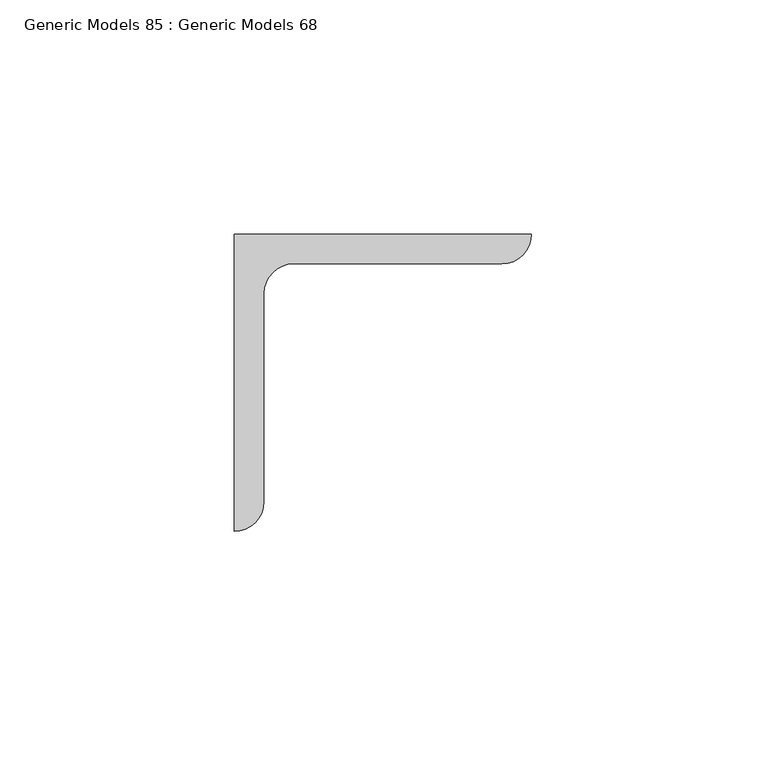
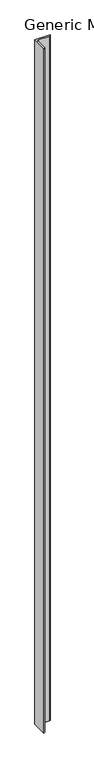
"""IFC4 building model written with IfcOpenShell, lengths in millimetres: proxy geometry, Generic Models 85 : Generic Models 68."""

from ifc_helpers import new_model, si_unit, point, frame, frame_2d, origin, place, context, project, spatial, polyline, circle_curve, trimmed, segment, composite_curve, outline, extrude, source, transform, mapped, element, save


def generic_models_85_generic_models_68_ff43cc48(model_context):
    return source(origin(), model_context, "Body", "SweptSolid", [
        extrude(outline(composite_curve([segment(polyline([(20530.4116945, 18496.0264581), (20593.9116945, 18496.0264581)]), True, "CONTINUOUS"), segment(trimmed(circle_curve(frame_2d((20587.5616945, 18496.0264581)), 6.35), [point((20593.9116945, 18496.0264581))], [point((20587.5616945, 18489.6764581))], False, "CARTESIAN"), True, "CONTINUOUS"), segment(polyline([(20587.5616945, 18489.6764581), (20543.1116945, 18489.6764581)]), True, "CONTINUOUS"), segment(trimmed(circle_curve(frame_2d((20543.1116945, 18483.3264581)), 6.35), [point((20543.1116945, 18489.6764581))], [point((20536.7616945, 18483.3264581))], True, "CARTESIAN"), True, "CONTINUOUS"), segment(polyline([(20536.7616945, 18483.3264581), (20536.7616945, 18438.8764581)]), True, "CONTINUOUS"), segment(trimmed(circle_curve(frame_2d((20530.4116945, 18438.8764581)), 6.35), [point((20536.7616945, 18438.8764581))], [point((20530.4116945, 18432.5264581))], False, "CARTESIAN"), True, "CONTINUOUS"), segment(polyline([(20530.4116945, 18432.5264581), (20530.4116945, 18496.0264581)]), True, "CONTINUOUS")], self_intersect=False)), frame((0.0, 0.0, 264380.6186948), z_axis=(0.0, 0.0, 1.0), x_axis=(1.0, 0.0, 0.0)), (0.0, 0.0, 1.0), 3006.09),
    ])


if __name__ == "__main__":
    model = new_model("IFC4")
    model_context = context("Model", 3, world=origin())
    ifc_project = project(units=[si_unit("LENGTHUNIT", "METRE", prefix="MILLI")], contexts=[model_context])
    site = spatial("IfcSite", under=ifc_project)
    building = spatial("IfcBuilding", under=site)
    placement = place(None, origin())
    generic_models_85_generic_models_68_shape = generic_models_85_generic_models_68_ff43cc48(model_context)
    element("IfcBuildingElementProxy", 1, Name="Generic Models 85 : Generic Models 68", ObjectType="Generic Models 85 : Generic Models 68", at=placement, inside=building, context=model_context, shape_type="MappedRepresentation", body=[
        mapped(generic_models_85_generic_models_68_shape, transform((0.0, 0.0, 0.0), x_axis=(1.0, 0.0, 0.0), y_axis=(0.0, 1.0, 0.0), z_axis=(0.0, 0.0, 1.0))),
    ])
    save(model, "model.ifc")

# Revit data of these elements
# Element 1 (IfcBuildingElementProxy, "Generic Models 85 : Generic Models 68")
#   Materials on its faces: "MAIN FENCE POST: (2) BACK/BACK GALVANIZED ANGLES (2) L2 1/2 X 2 1/2 X 1/4\") ANCHORED TO 8\"W X 42\" DEEP CONCRETE FOOTING(1)"
# Materials
#   "MAIN FENCE POST: (2) BACK/BACK GALVANIZED ANGLES (2) L2 1/2 X 2 1/2 X 1/4\") ANCHORED TO 8\"W X 42\" DEEP CONCRETE FOOTING(1)": class "Unassigned", colour RGB 211 211 211, transparency 0, Cost = 0
